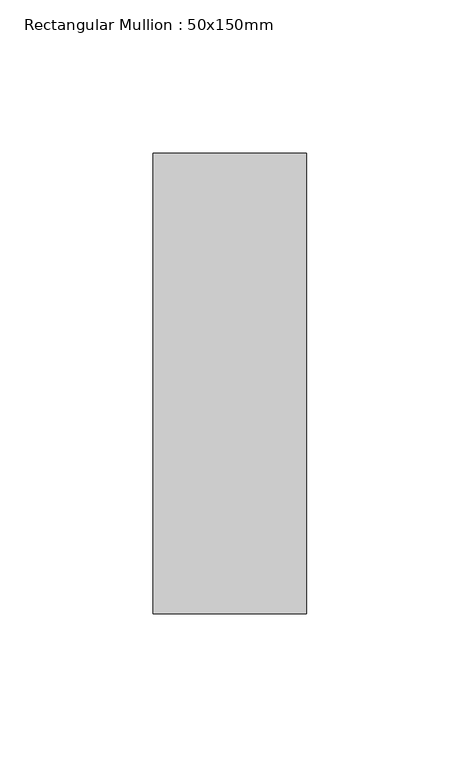
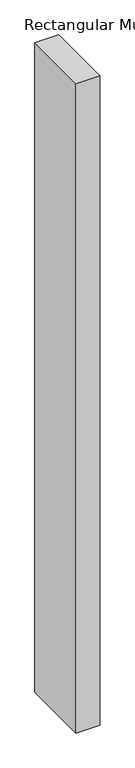
"""IFC4 building model written with IfcOpenShell, lengths in millimetres: member geometry, Rectangular Mullion : 50x150mm."""

import ifcopenshell
import ifcopenshell.guid

model = None  # the IFC model being written
_history = None  # IfcOwnerHistory: only IFC2X3 demands one
_inside = {}  # id of a spatial element -> (the spatial element, [elements in it])
_under = {}  # id of a project, library or spatial element -> (it, [spatial elements below it])
_declared = {}  # id of a project -> (the project, [libraries it declares])
_typed = {}  # id of a type object -> (the type object, [elements of that type])
_made_of = {}  # id of a material, layer set ... -> (it, [elements and type objects made of it])


def new_model(schema):
    """Start an empty IFC model of exactly this schema.

    Asked for "IFC4X3", IfcOpenShell would pick the latest addendum, in which some entities
    have other attributes; the version numbers below select the first issue.
    IFC2X3 requires an IfcOwnerHistory on every rooted entity: one is made here for all.
    """
    global model, _history
    if schema == "IFC4X3":
        model = ifcopenshell.file(schema_version=(4, 3, 0, 0))
    else:
        model = ifcopenshell.file(schema=schema)
    _inside.clear()
    _under.clear()
    _declared.clear()
    _typed.clear()
    _made_of.clear()
    _history = None
    if model.schema == "IFC2X3":
        org = make("IfcOrganization", Name="unknown")
        user = make(
            "IfcPersonAndOrganization",
            ThePerson=make("IfcPerson", FamilyName="unknown"),
            TheOrganization=org,
        )
        app = make(
            "IfcApplication",
            ApplicationDeveloper=org,
            Version="unknown",
            ApplicationFullName="unknown",
            ApplicationIdentifier="unknown",
        )
        _history = make(
            "IfcOwnerHistory",
            OwningUser=user,
            OwningApplication=app,
            ChangeAction="ADDED",
            CreationDate=0,
        )
    return model


def make(cls, **values):
    """One entity of the class cls with the attributes given. An attribute that is None is left unset."""
    return model.create_entity(
        cls, **{name: value for name, value in values.items() if value is not None}
    )


def rooted(cls, **values):
    """An entity with a GlobalId (a new one), such as an element, a storey or a relation."""
    return make(cls, GlobalId=ifcopenshell.guid.new(), OwnerHistory=_history, **values)


def si_unit(unit_type, name, prefix=None):
    """IfcSIUnit, for example si_unit("LENGTHUNIT", "METRE", prefix="MILLI")."""
    return make("IfcSIUnit", UnitType=unit_type, Prefix=prefix, Name=name)


def assignment(units):
    """IfcUnitAssignment: the units of a project."""
    return None if units is None else make("IfcUnitAssignment", Units=units)


def point(xyz):
    """IfcCartesianPoint."""
    return None if xyz is None else make("IfcCartesianPoint", Coordinates=xyz)


def direction(xyz):
    """IfcDirection."""
    return None if xyz is None else make("IfcDirection", DirectionRatios=xyz)


def frame(location, z_axis=None, x_axis=None):
    """IfcAxis2Placement3D, a coordinate frame: its origin and axes. An axis left out is left unset."""
    return make(
        "IfcAxis2Placement3D",
        Location=point(location),
        Axis=direction(z_axis),
        RefDirection=direction(x_axis),
    )


def origin():
    """The frame at (0, 0, 0) with its axes left unset."""
    return frame((0.0, 0.0, 0.0))


def place(relative_to, where):
    """IfcLocalPlacement: puts the frame where relative to a parent placement (None: the world)."""
    return make(
        "IfcLocalPlacement", PlacementRelTo=relative_to, RelativePlacement=where
    )


def context(
    kind, dimensions, precision=None, world=None, true_north=None, identifier=None
):
    """IfcGeometricRepresentationContext, for example the 3D "Model" context."""
    return make(
        "IfcGeometricRepresentationContext",
        ContextIdentifier=identifier,
        ContextType=kind,
        CoordinateSpaceDimension=dimensions,
        Precision=precision,
        WorldCoordinateSystem=world,
        TrueNorth=true_north,
    )


def project(units=None, contexts=None):
    """IfcProject with its units and contexts."""
    return rooted(
        "IfcProject",
        Name="project",
        RepresentationContexts=contexts,
        UnitsInContext=assignment(units),
    )


def spatial(cls, under=None, at=None, **own):
    """A site, building, storey or space (cls), placed at a placement, below another one or the project."""
    s = rooted(cls, ObjectPlacement=at, **own)
    if under is not None:
        _under.setdefault(under.id(), (under, []))[1].append(s)
    return s


def polyline(points):
    """IfcPolyline through the points."""
    return make("IfcPolyline", Points=[point(p) for p in points])


def outline(outer, holes=None, kind="AREA"):
    """IfcArbitraryClosedProfileDef: a profile drawn as a closed curve; with holes, ...WithVoids."""
    if holes is None:
        return make("IfcArbitraryClosedProfileDef", ProfileType=kind, OuterCurve=outer)
    return make(
        "IfcArbitraryProfileDefWithVoids",
        ProfileType=kind,
        OuterCurve=outer,
        InnerCurves=holes,
    )


def extrude(swept, where, along, depth):
    """IfcExtrudedAreaSolid: the profile swept, set in the frame where, extruded along a direction by depth."""
    return make(
        "IfcExtrudedAreaSolid",
        SweptArea=swept,
        Position=where,
        ExtrudedDirection=direction(along),
        Depth=depth,
    )


def shape(context_of_items, identifier, shape_type, items):
    """IfcShapeRepresentation: the items that make up one representation, for example the "Body"."""
    return make(
        "IfcShapeRepresentation",
        ContextOfItems=context_of_items,
        RepresentationIdentifier=identifier,
        RepresentationType=shape_type,
        Items=items,
    )


def source(mapping_origin, context_of_items, identifier, shape_type, items):
    """IfcRepresentationMap: a shape defined once, which mapped items show again and again."""
    return make(
        "IfcRepresentationMap",
        MappingOrigin=mapping_origin,
        MappedRepresentation=shape(context_of_items, identifier, shape_type, items),
    )


def transform(
    local_origin,
    x_axis=None,
    y_axis=None,
    z_axis=None,
    scale=None,
    scale2=None,
    scale3=None,
    uniform=True,
):
    """IfcCartesianTransformationOperator3D, or its non-uniform kind. x_axis, y_axis, z_axis: its Axis1, 2, 3."""
    if uniform:
        return make(
            "IfcCartesianTransformationOperator3D",
            Axis1=direction(x_axis),
            Axis2=direction(y_axis),
            LocalOrigin=point(local_origin),
            Scale=scale,
            Axis3=direction(z_axis),
        )
    return make(
        "IfcCartesianTransformationOperator3DnonUniform",
        Axis1=direction(x_axis),
        Axis2=direction(y_axis),
        LocalOrigin=point(local_origin),
        Scale=scale,
        Axis3=direction(z_axis),
        Scale2=scale2,
        Scale3=scale3,
    )


def mapped(mapping_source, mapping_target):
    """IfcMappedItem: shows the shape of a source again, moved by a transform."""
    return make(
        "IfcMappedItem", MappingSource=mapping_source, MappingTarget=mapping_target
    )


def made_of(thing, what):
    """Note that an element or type object is made of a material, layer set ...; save() writes the relation."""
    if what is not None:
        _made_of.setdefault(what.id(), (what, []))[1].append(thing)
    return thing


def element(
    cls,
    number,
    at=None,
    inside=None,
    cuts=None,
    type_object=None,
    material=None,
    context=None,
    identifier="Body",
    shape_type=None,
    held_by="IfcProductDefinitionShape",
    body=None,
    shapes=None,
    **own,
):
    """One element of the class cls, such as IfcWall. Its Tag is "e" and its number.

    at: its placement. inside: the storey or other place that contains it. cuts: it is an
    opening in that element (IfcRelVoidsElement). A single representation is given by context,
    identifier, shape_type and body (its items); several are given by shapes. held_by: the class
    of the entity that holds the representations. save() writes the other relations.
    """
    e = rooted(cls, Tag="e%d" % number, ObjectPlacement=at, **own)
    if body is not None:
        shapes = [shape(context, identifier, shape_type, body)]
    if shapes is not None:
        e.Representation = make(held_by, Representations=shapes)
    if inside is not None:
        _inside.setdefault(inside.id(), (inside, []))[1].append(e)
    if cuts is not None:
        rooted(
            "IfcRelVoidsElement", RelatingBuildingElement=cuts, RelatedOpeningElement=e
        )
    if type_object is not None:
        _typed.setdefault(type_object.id(), (type_object, []))[1].append(e)
    return made_of(e, material)


def aggregate(whole, parts):
    """IfcRelAggregates: a whole, such as a stair, and the parts it consists of."""
    return rooted("IfcRelAggregates", RelatingObject=whole, RelatedObjects=parts)


def save(model, path):
    """Write the relations noted so far, then the file.

    IfcRelAggregates (storeys below a building ...), IfcRelContainedInSpatialStructure (elements
    in a storey), IfcRelDefinesByType, IfcRelAssociatesMaterial and IfcRelDeclares: one each for
    every whole, place, type object, material and project.
    """
    for whole, parts in _under.values():
        aggregate(whole, parts)
    for where, things in _inside.values():
        rooted(
            "IfcRelContainedInSpatialStructure",
            RelatedElements=things,
            RelatingStructure=where,
        )
    for kind, things in _typed.values():
        rooted("IfcRelDefinesByType", RelatedObjects=things, RelatingType=kind)
    for what, things in _made_of.values():
        rooted("IfcRelAssociatesMaterial", RelatedObjects=things, RelatingMaterial=what)
    for by, libraries in _declared.values():
        rooted("IfcRelDeclares", RelatingContext=by, RelatedDefinitions=libraries)
    model.write(path)


def rectangular_mullion_50x150mm_f6f7edf2(model_context):
    return source(origin(), model_context, "Body", "SweptSolid", [
        extrude(outline(polyline([(25.0, 75.0), (25.0, -75.0), (-25.0, -75.0), (-25.0, 75.0), (25.0, 75.0)])), frame((0.0, 0.0, -1449.9999998), z_axis=(0.0, 0.0, 1.0), x_axis=(1.0, 0.0, 0.0)), (0.0, 0.0, 1.0), 1449.9999998),
    ])


if __name__ == "__main__":
    model = new_model("IFC4")
    model_context = context("Model", 3, world=origin())
    ifc_project = project(units=[si_unit("LENGTHUNIT", "METRE", prefix="MILLI")], contexts=[model_context])
    site = spatial("IfcSite", under=ifc_project)
    building = spatial("IfcBuilding", under=site)
    placement = place(None, origin())
    rectangular_mullion_50x150mm_shape = rectangular_mullion_50x150mm_f6f7edf2(model_context)
    element("IfcMember", 1, ObjectType="Rectangular Mullion : 50x150mm", at=placement, inside=building, context=model_context, shape_type="MappedRepresentation", body=[
        mapped(rectangular_mullion_50x150mm_shape, transform((0.0, 0.0, 0.0), x_axis=(1.0, 0.0, 0.0), y_axis=(0.0, 1.0, 0.0), z_axis=(0.0, 0.0, 1.0))),
    ])
    save(model, "model.ifc")

# Revit data of these elements
# Type "Rectangular Mullion : 50x150mm"
#   Keynote = "H11"
#   built-in parameter 1007304 = 0.492126 (stored number, unit not read)
#   built-in parameter 1007301 = 0.082021 (stored number, unit not read)
#   built-in parameter 1007300 = 0.082021 (stored number, unit not read)
# Element 1 (IfcMember, "Rectangular Mullion : 50x150mm")
#   Materials on its faces: "Aluminium"
# Materials
#   "Aluminium": class "Metal", colour RGB 247 247 247, transparency 0, Description = "Aluminium 6061", Cost = 0
